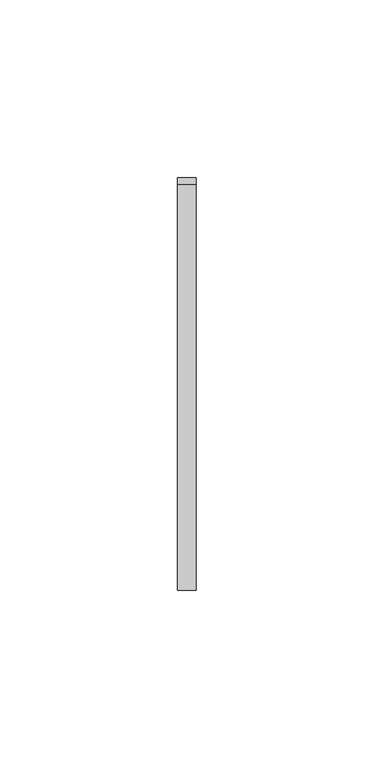
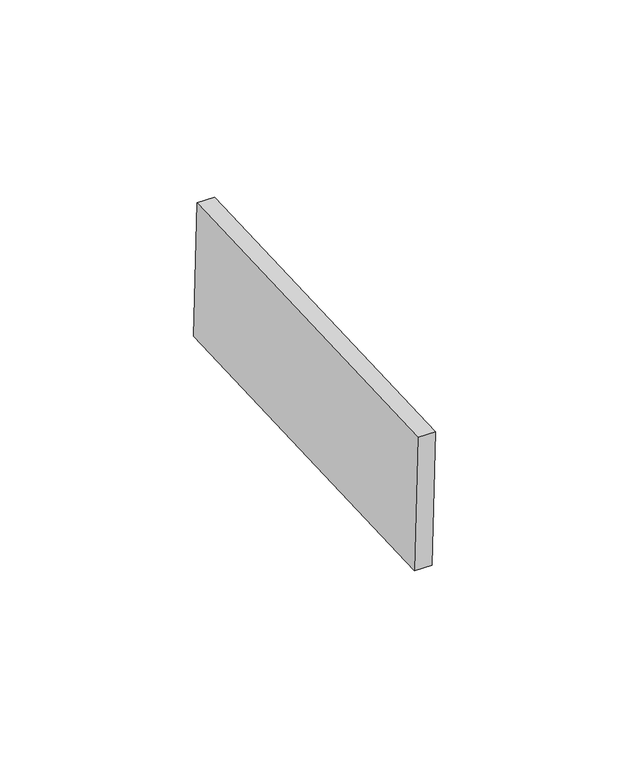
"""IFC4 building model written with IfcOpenShell, lengths in millimetres: proxy geometry, Inner panel:Inner panel:1:Inner panel:1 : Inner panel:Inner panel:300324:2:Inner panel:1:Inner panel:1 : Inner panel:Inner panel:300324:2 : Inner panel:Inner panel:1:Inner panel:1 : Inner panel:Inner panel:300324:300043:63 : Inner panel:Inner panel:1:Inner panel:1 : Inner panel:Inner panel:300324:2:Inner panel:1:Inner panel:1 : Inner panel:Inner panel:300324:2 : Inner panel:Inner panel:1:Inner panel:1 : Inner panel:Inner panel:300324:300043:308120."""

from ifc_helpers import new_model, si_unit, frame, origin, place, context, project, spatial, polyline, outline, extrude, source, transform, mapped, element, save


def generic_models_51c1b564(model_context):
    return source(origin(), model_context, "Body", "SweptSolid", [
        extrude(outline(polyline([(0.0, -114.2999999), (0.0, 0.0), (5.2138089, 0.0), (5.2138089, -114.2999999), (0.0, -114.2999999)])), frame((593530.195117, -569006.6262918, 8772.0084398), z_axis=(0.0, -0.04163054471215927, 0.9991330730923529), x_axis=(-1.0, 0.0, 0.0)), (0.0, 0.0, 1.0), 43.2233908),
    ])


if __name__ == "__main__":
    model = new_model("IFC4")
    model_context = context("Model", 3, world=origin())
    ifc_project = project(units=[si_unit("LENGTHUNIT", "METRE", prefix="MILLI")], contexts=[model_context])
    site = spatial("IfcSite", under=ifc_project)
    building = spatial("IfcBuilding", under=site)
    placement = place(None, origin())
    generic_models_shape = generic_models_51c1b564(model_context)
    element("IfcBuildingElementProxy", 1, Name="Inner panel:Inner panel:1:Inner panel:1 : Inner panel:Inner panel:300324:2:Inner panel:1:Inner panel:1 : Inner panel:Inner panel:300324:2 : Inner panel:Inner panel:1:Inner panel:1 : Inner panel:Inner panel:300324:300043:63 : Inner panel:Inner panel:1:Inner panel:1 : Inner panel:Inner panel:300324:2:Inner panel:1:Inner panel:1 : Inner panel:Inner panel:300324:2 : Inner panel:Inner panel:1:Inner panel:1 : Inner panel:Inner panel:300324:300043:308120", ObjectType="Inner panel:Inner panel:1:Inner panel:1 : Inner panel:Inner panel:300324:2:Inner panel:1:Inner panel:1 : Inner panel:Inner panel:300324:2 : Inner panel:Inner panel:1:Inner panel:1 : Inner panel:Inner panel:300324:300043:63 : Inner panel:Inner panel:1:Inner panel:1 : Inner panel:Inner panel:300324:2:Inner panel:1:Inner panel:1 : Inner panel:Inner panel:300324:2 : Inner panel:Inner panel:1:Inner panel:1 : Inner panel:Inner panel:300324:300043:308120", at=placement, inside=building, context=model_context, shape_type="MappedRepresentation", body=[
        mapped(generic_models_shape, transform((0.0, 0.0, 0.0), x_axis=(1.0, 0.0, 0.0), y_axis=(0.0, 1.0, 0.0), z_axis=(0.0, 0.0, 1.0))),
    ])
    save(model, "model.ifc")

# Revit data of these elements
# Type "Inner panel:Inner panel:1:Inner panel:1 : Inner panel:Inner panel:300324:2:Inner panel:1:Inner panel:1 : Inner panel:Inner panel:300324:2 : Inner panel:Inner panel:1:Inner panel:1 : Inner panel:Inner panel:300324:300043:63 : Inner panel:Inner panel:1:Inner panel:1 : Inner panel:Inner panel:300324:2:Inner panel:1:Inner panel:1 : Inner panel:Inner panel:300324:2 : Inner panel:Inner panel:1:Inner panel:1 : Inner panel:Inner panel:300324:300043:308120"
#   NameOverride = "Inner panel:Inner panel:1:Inner panel:1 : Inner panel:Inner panel:300324:2:Inner panel:1:Inner panel:1 : Inner panel:Inner panel:300324:2 : Inner panel:Inner panel:1:Inner panel:1 : Inner panel:Inner panel:300324:300043:308120"
#   ObjectTypeOverride = "Inner panel:1:Inner panel:1 : Inner panel:Inner panel:300324:2 : Inner panel:Inner panel:1:Inner panel:1 : Inner panel:Inner panel:300324:300043"
#   Reference = "Inner panel"
#   Tag = "308120"
# Element 1 (IfcBuildingElementProxy, "Inner panel:Inner panel:1:Inner panel:1 : Inner panel:Inner panel:300324:2:Inner panel:1:Inner panel:1 : Inner panel:Inner panel:300324:2 : Inner panel:Inner panel:1:Inner panel:1 : Inner panel:Inner panel:300324:300043:63 : Inner panel:Inner panel:1:Inner panel:1 : Inner panel:Inner panel:300324:2:Inner panel:1:Inner panel:1 : Inner panel:Inner panel:300324:2 : Inner panel:Inner panel:1:Inner panel:1 : Inner panel:Inner panel:300324:300043:308120")
#   Materials on its faces: "SLIDING CLIP"
# Materials
#   "SLIDING CLIP": class "Generic", colour RGB 120 120 120, transparency 0, Cost = 0
